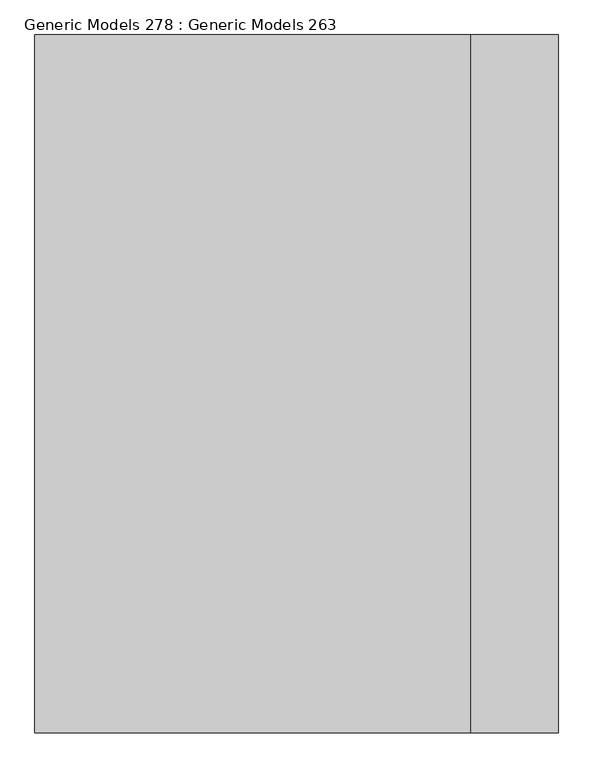
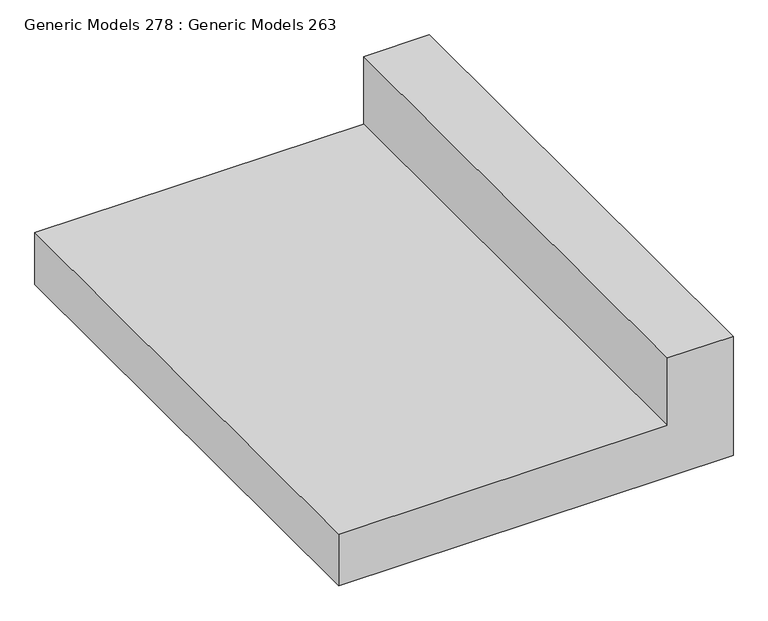
"""IFC4 building model written with IfcOpenShell, lengths in millimetres: proxy geometry, Generic Models 278 : Generic Models 263."""

import ifcopenshell
import ifcopenshell.guid

model = None  # the IFC model being written
_history = None  # IfcOwnerHistory: only IFC2X3 demands one
_inside = {}  # id of a spatial element -> (the spatial element, [elements in it])
_under = {}  # id of a project, library or spatial element -> (it, [spatial elements below it])
_declared = {}  # id of a project -> (the project, [libraries it declares])
_typed = {}  # id of a type object -> (the type object, [elements of that type])
_made_of = {}  # id of a material, layer set ... -> (it, [elements and type objects made of it])


def new_model(schema):
    """Start an empty IFC model of exactly this schema.

    Asked for "IFC4X3", IfcOpenShell would pick the latest addendum, in which some entities
    have other attributes; the version numbers below select the first issue.
    IFC2X3 requires an IfcOwnerHistory on every rooted entity: one is made here for all.
    """
    global model, _history
    if schema == "IFC4X3":
        model = ifcopenshell.file(schema_version=(4, 3, 0, 0))
    else:
        model = ifcopenshell.file(schema=schema)
    _inside.clear()
    _under.clear()
    _declared.clear()
    _typed.clear()
    _made_of.clear()
    _history = None
    if model.schema == "IFC2X3":
        org = make("IfcOrganization", Name="unknown")
        user = make(
            "IfcPersonAndOrganization",
            ThePerson=make("IfcPerson", FamilyName="unknown"),
            TheOrganization=org,
        )
        app = make(
            "IfcApplication",
            ApplicationDeveloper=org,
            Version="unknown",
            ApplicationFullName="unknown",
            ApplicationIdentifier="unknown",
        )
        _history = make(
            "IfcOwnerHistory",
            OwningUser=user,
            OwningApplication=app,
            ChangeAction="ADDED",
            CreationDate=0,
        )
    return model


def make(cls, **values):
    """One entity of the class cls with the attributes given. An attribute that is None is left unset."""
    return model.create_entity(
        cls, **{name: value for name, value in values.items() if value is not None}
    )


def rooted(cls, **values):
    """An entity with a GlobalId (a new one), such as an element, a storey or a relation."""
    return make(cls, GlobalId=ifcopenshell.guid.new(), OwnerHistory=_history, **values)


def si_unit(unit_type, name, prefix=None):
    """IfcSIUnit, for example si_unit("LENGTHUNIT", "METRE", prefix="MILLI")."""
    return make("IfcSIUnit", UnitType=unit_type, Prefix=prefix, Name=name)


def assignment(units):
    """IfcUnitAssignment: the units of a project."""
    return None if units is None else make("IfcUnitAssignment", Units=units)


def point(xyz):
    """IfcCartesianPoint."""
    return None if xyz is None else make("IfcCartesianPoint", Coordinates=xyz)


def direction(xyz):
    """IfcDirection."""
    return None if xyz is None else make("IfcDirection", DirectionRatios=xyz)


def frame(location, z_axis=None, x_axis=None):
    """IfcAxis2Placement3D, a coordinate frame: its origin and axes. An axis left out is left unset."""
    return make(
        "IfcAxis2Placement3D",
        Location=point(location),
        Axis=direction(z_axis),
        RefDirection=direction(x_axis),
    )


def origin():
    """The frame at (0, 0, 0) with its axes left unset."""
    return frame((0.0, 0.0, 0.0))


def place(relative_to, where):
    """IfcLocalPlacement: puts the frame where relative to a parent placement (None: the world)."""
    return make(
        "IfcLocalPlacement", PlacementRelTo=relative_to, RelativePlacement=where
    )


def context(
    kind, dimensions, precision=None, world=None, true_north=None, identifier=None
):
    """IfcGeometricRepresentationContext, for example the 3D "Model" context."""
    return make(
        "IfcGeometricRepresentationContext",
        ContextIdentifier=identifier,
        ContextType=kind,
        CoordinateSpaceDimension=dimensions,
        Precision=precision,
        WorldCoordinateSystem=world,
        TrueNorth=true_north,
    )


def project(units=None, contexts=None):
    """IfcProject with its units and contexts."""
    return rooted(
        "IfcProject",
        Name="project",
        RepresentationContexts=contexts,
        UnitsInContext=assignment(units),
    )


def spatial(cls, under=None, at=None, **own):
    """A site, building, storey or space (cls), placed at a placement, below another one or the project."""
    s = rooted(cls, ObjectPlacement=at, **own)
    if under is not None:
        _under.setdefault(under.id(), (under, []))[1].append(s)
    return s


def polyline(points):
    """IfcPolyline through the points."""
    return make("IfcPolyline", Points=[point(p) for p in points])


def outline(outer, holes=None, kind="AREA"):
    """IfcArbitraryClosedProfileDef: a profile drawn as a closed curve; with holes, ...WithVoids."""
    if holes is None:
        return make("IfcArbitraryClosedProfileDef", ProfileType=kind, OuterCurve=outer)
    return make(
        "IfcArbitraryProfileDefWithVoids",
        ProfileType=kind,
        OuterCurve=outer,
        InnerCurves=holes,
    )


def extrude(swept, where, along, depth):
    """IfcExtrudedAreaSolid: the profile swept, set in the frame where, extruded along a direction by depth."""
    return make(
        "IfcExtrudedAreaSolid",
        SweptArea=swept,
        Position=where,
        ExtrudedDirection=direction(along),
        Depth=depth,
    )


def shape(context_of_items, identifier, shape_type, items):
    """IfcShapeRepresentation: the items that make up one representation, for example the "Body"."""
    return make(
        "IfcShapeRepresentation",
        ContextOfItems=context_of_items,
        RepresentationIdentifier=identifier,
        RepresentationType=shape_type,
        Items=items,
    )


def source(mapping_origin, context_of_items, identifier, shape_type, items):
    """IfcRepresentationMap: a shape defined once, which mapped items show again and again."""
    return make(
        "IfcRepresentationMap",
        MappingOrigin=mapping_origin,
        MappedRepresentation=shape(context_of_items, identifier, shape_type, items),
    )


def transform(
    local_origin,
    x_axis=None,
    y_axis=None,
    z_axis=None,
    scale=None,
    scale2=None,
    scale3=None,
    uniform=True,
):
    """IfcCartesianTransformationOperator3D, or its non-uniform kind. x_axis, y_axis, z_axis: its Axis1, 2, 3."""
    if uniform:
        return make(
            "IfcCartesianTransformationOperator3D",
            Axis1=direction(x_axis),
            Axis2=direction(y_axis),
            LocalOrigin=point(local_origin),
            Scale=scale,
            Axis3=direction(z_axis),
        )
    return make(
        "IfcCartesianTransformationOperator3DnonUniform",
        Axis1=direction(x_axis),
        Axis2=direction(y_axis),
        LocalOrigin=point(local_origin),
        Scale=scale,
        Axis3=direction(z_axis),
        Scale2=scale2,
        Scale3=scale3,
    )


def mapped(mapping_source, mapping_target):
    """IfcMappedItem: shows the shape of a source again, moved by a transform."""
    return make(
        "IfcMappedItem", MappingSource=mapping_source, MappingTarget=mapping_target
    )


def made_of(thing, what):
    """Note that an element or type object is made of a material, layer set ...; save() writes the relation."""
    if what is not None:
        _made_of.setdefault(what.id(), (what, []))[1].append(thing)
    return thing


def element(
    cls,
    number,
    at=None,
    inside=None,
    cuts=None,
    type_object=None,
    material=None,
    context=None,
    identifier="Body",
    shape_type=None,
    held_by="IfcProductDefinitionShape",
    body=None,
    shapes=None,
    **own,
):
    """One element of the class cls, such as IfcWall. Its Tag is "e" and its number.

    at: its placement. inside: the storey or other place that contains it. cuts: it is an
    opening in that element (IfcRelVoidsElement). A single representation is given by context,
    identifier, shape_type and body (its items); several are given by shapes. held_by: the class
    of the entity that holds the representations. save() writes the other relations.
    """
    e = rooted(cls, Tag="e%d" % number, ObjectPlacement=at, **own)
    if body is not None:
        shapes = [shape(context, identifier, shape_type, body)]
    if shapes is not None:
        e.Representation = make(held_by, Representations=shapes)
    if inside is not None:
        _inside.setdefault(inside.id(), (inside, []))[1].append(e)
    if cuts is not None:
        rooted(
            "IfcRelVoidsElement", RelatingBuildingElement=cuts, RelatedOpeningElement=e
        )
    if type_object is not None:
        _typed.setdefault(type_object.id(), (type_object, []))[1].append(e)
    return made_of(e, material)


def aggregate(whole, parts):
    """IfcRelAggregates: a whole, such as a stair, and the parts it consists of."""
    return rooted("IfcRelAggregates", RelatingObject=whole, RelatedObjects=parts)


def save(model, path):
    """Write the relations noted so far, then the file.

    IfcRelAggregates (storeys below a building ...), IfcRelContainedInSpatialStructure (elements
    in a storey), IfcRelDefinesByType, IfcRelAssociatesMaterial and IfcRelDeclares: one each for
    every whole, place, type object, material and project.
    """
    for whole, parts in _under.values():
        aggregate(whole, parts)
    for where, things in _inside.values():
        rooted(
            "IfcRelContainedInSpatialStructure",
            RelatedElements=things,
            RelatingStructure=where,
        )
    for kind, things in _typed.values():
        rooted("IfcRelDefinesByType", RelatedObjects=things, RelatingType=kind)
    for what, things in _made_of.values():
        rooted("IfcRelAssociatesMaterial", RelatedObjects=things, RelatingMaterial=what)
    for by, libraries in _declared.values():
        rooted("IfcRelDeclares", RelatingContext=by, RelatedDefinitions=libraries)
    model.write(path)


def generic_models_278_generic_models_263_5a7632f5(model_context):
    return source(origin(), model_context, "Body", "SweptSolid", [
        extrude(outline(polyline([(-381.0, 60947.5797726), (-381.0, 60185.5797726), (-508.0, 60185.5797726), (-508.0, 61099.9797726), (-215.9, 61099.9797726), (-215.9, 60947.5797726), (-381.0, 60947.5797726)])), frame((0.0, -94.4486541, 0.0), z_axis=(0.0, 1.0, 0.0), x_axis=(0.0, 0.0, 1.0)), (0.0, 0.0, 1.0), 1219.2),
    ])


if __name__ == "__main__":
    model = new_model("IFC4")
    model_context = context("Model", 3, world=origin())
    ifc_project = project(units=[si_unit("LENGTHUNIT", "METRE", prefix="MILLI")], contexts=[model_context])
    site = spatial("IfcSite", under=ifc_project)
    building = spatial("IfcBuilding", under=site)
    placement = place(None, origin())
    generic_models_278_generic_models_263_shape = generic_models_278_generic_models_263_5a7632f5(model_context)
    element("IfcBuildingElementProxy", 1, Name="Generic Models 278 : Generic Models 263", ObjectType="Generic Models 278 : Generic Models 263", at=placement, inside=building, context=model_context, shape_type="MappedRepresentation", body=[
        mapped(generic_models_278_generic_models_263_shape, transform((0.0, 0.0, 0.0), x_axis=(1.0, 0.0, 0.0), y_axis=(0.0, 1.0, 0.0), z_axis=(0.0, 0.0, 1.0))),
    ])
    save(model, "model.ifc")

# Revit data of these elements
# Element 1 (IfcBuildingElementProxy, "Generic Models 278 : Generic Models 263")
#   Materials on its faces: "5\" MIN. COMPACTED BASE AGGREGATE UNDER CURB"
# Materials
#   "5\" MIN. COMPACTED BASE AGGREGATE UNDER CURB": class "Miscellaneous", colour RGB 183 184 198, transparency 0, Cost = 0
